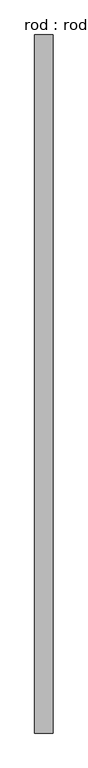
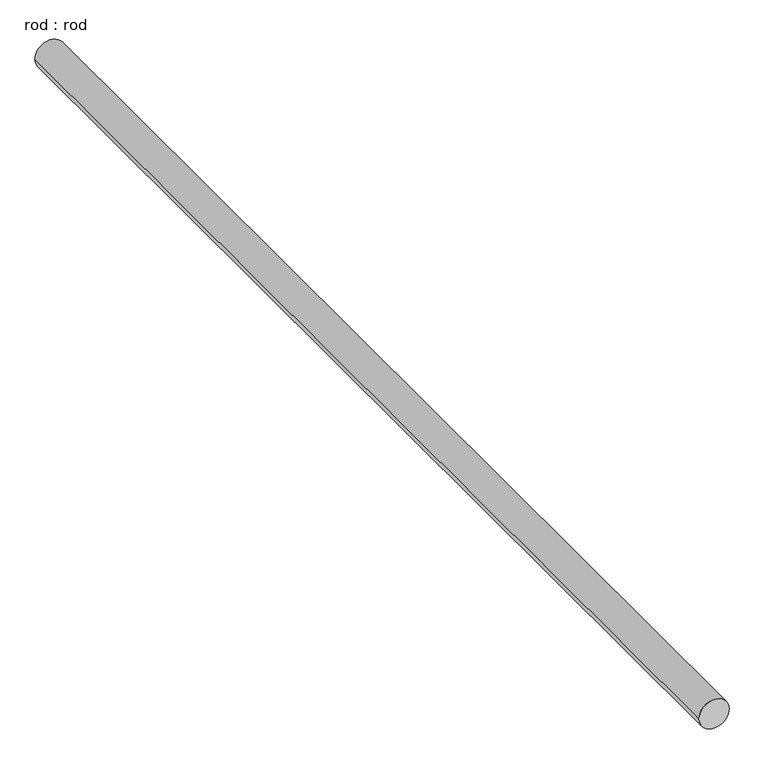
"""IFC4 building model written with IfcOpenShell, lengths in millimetres: proxy geometry, rod : rod."""

import ifcopenshell
import ifcopenshell.guid

model = None  # the IFC model being written
_history = None  # IfcOwnerHistory: only IFC2X3 demands one
_inside = {}  # id of a spatial element -> (the spatial element, [elements in it])
_under = {}  # id of a project, library or spatial element -> (it, [spatial elements below it])
_declared = {}  # id of a project -> (the project, [libraries it declares])
_typed = {}  # id of a type object -> (the type object, [elements of that type])
_made_of = {}  # id of a material, layer set ... -> (it, [elements and type objects made of it])


def new_model(schema):
    """Start an empty IFC model of exactly this schema.

    Asked for "IFC4X3", IfcOpenShell would pick the latest addendum, in which some entities
    have other attributes; the version numbers below select the first issue.
    IFC2X3 requires an IfcOwnerHistory on every rooted entity: one is made here for all.
    """
    global model, _history
    if schema == "IFC4X3":
        model = ifcopenshell.file(schema_version=(4, 3, 0, 0))
    else:
        model = ifcopenshell.file(schema=schema)
    _inside.clear()
    _under.clear()
    _declared.clear()
    _typed.clear()
    _made_of.clear()
    _history = None
    if model.schema == "IFC2X3":
        org = make("IfcOrganization", Name="unknown")
        user = make(
            "IfcPersonAndOrganization",
            ThePerson=make("IfcPerson", FamilyName="unknown"),
            TheOrganization=org,
        )
        app = make(
            "IfcApplication",
            ApplicationDeveloper=org,
            Version="unknown",
            ApplicationFullName="unknown",
            ApplicationIdentifier="unknown",
        )
        _history = make(
            "IfcOwnerHistory",
            OwningUser=user,
            OwningApplication=app,
            ChangeAction="ADDED",
            CreationDate=0,
        )
    return model


def make(cls, **values):
    """One entity of the class cls with the attributes given. An attribute that is None is left unset."""
    return model.create_entity(
        cls, **{name: value for name, value in values.items() if value is not None}
    )


def rooted(cls, **values):
    """An entity with a GlobalId (a new one), such as an element, a storey or a relation."""
    return make(cls, GlobalId=ifcopenshell.guid.new(), OwnerHistory=_history, **values)


def si_unit(unit_type, name, prefix=None):
    """IfcSIUnit, for example si_unit("LENGTHUNIT", "METRE", prefix="MILLI")."""
    return make("IfcSIUnit", UnitType=unit_type, Prefix=prefix, Name=name)


def assignment(units):
    """IfcUnitAssignment: the units of a project."""
    return None if units is None else make("IfcUnitAssignment", Units=units)


def point(xyz):
    """IfcCartesianPoint."""
    return None if xyz is None else make("IfcCartesianPoint", Coordinates=xyz)


def direction(xyz):
    """IfcDirection."""
    return None if xyz is None else make("IfcDirection", DirectionRatios=xyz)


def frame(location, z_axis=None, x_axis=None):
    """IfcAxis2Placement3D, a coordinate frame: its origin and axes. An axis left out is left unset."""
    return make(
        "IfcAxis2Placement3D",
        Location=point(location),
        Axis=direction(z_axis),
        RefDirection=direction(x_axis),
    )


def frame_2d(location, x_axis=None):
    """IfcAxis2Placement2D, a coordinate frame in the plane: its origin and x axis."""
    return make(
        "IfcAxis2Placement2D", Location=point(location), RefDirection=direction(x_axis)
    )


def origin():
    """The frame at (0, 0, 0) with its axes left unset."""
    return frame((0.0, 0.0, 0.0))


def place(relative_to, where):
    """IfcLocalPlacement: puts the frame where relative to a parent placement (None: the world)."""
    return make(
        "IfcLocalPlacement", PlacementRelTo=relative_to, RelativePlacement=where
    )


def context(
    kind, dimensions, precision=None, world=None, true_north=None, identifier=None
):
    """IfcGeometricRepresentationContext, for example the 3D "Model" context."""
    return make(
        "IfcGeometricRepresentationContext",
        ContextIdentifier=identifier,
        ContextType=kind,
        CoordinateSpaceDimension=dimensions,
        Precision=precision,
        WorldCoordinateSystem=world,
        TrueNorth=true_north,
    )


def project(units=None, contexts=None):
    """IfcProject with its units and contexts."""
    return rooted(
        "IfcProject",
        Name="project",
        RepresentationContexts=contexts,
        UnitsInContext=assignment(units),
    )


def spatial(cls, under=None, at=None, **own):
    """A site, building, storey or space (cls), placed at a placement, below another one or the project."""
    s = rooted(cls, ObjectPlacement=at, **own)
    if under is not None:
        _under.setdefault(under.id(), (under, []))[1].append(s)
    return s


def circle_curve(where, radius):
    """IfcCircle in the frame where."""
    return make("IfcCircle", Position=where, Radius=radius)


def trimmed(basis, trim1, trim2, sense, master):
    """IfcTrimmedCurve: the piece of a basis curve between two trims."""
    return make(
        "IfcTrimmedCurve",
        BasisCurve=basis,
        Trim1=trim1,
        Trim2=trim2,
        SenseAgreement=sense,
        MasterRepresentation=master,
    )


def segment(curve, same_sense, transition):
    """IfcCompositeCurveSegment."""
    return make(
        "IfcCompositeCurveSegment",
        Transition=transition,
        SameSense=same_sense,
        ParentCurve=curve,
    )


def composite_curve(segments, self_intersect=None):
    """IfcCompositeCurve: segments joined end to end."""
    return make("IfcCompositeCurve", Segments=segments, SelfIntersect=self_intersect)


def outline(outer, holes=None, kind="AREA"):
    """IfcArbitraryClosedProfileDef: a profile drawn as a closed curve; with holes, ...WithVoids."""
    if holes is None:
        return make("IfcArbitraryClosedProfileDef", ProfileType=kind, OuterCurve=outer)
    return make(
        "IfcArbitraryProfileDefWithVoids",
        ProfileType=kind,
        OuterCurve=outer,
        InnerCurves=holes,
    )


def extrude(swept, where, along, depth):
    """IfcExtrudedAreaSolid: the profile swept, set in the frame where, extruded along a direction by depth."""
    return make(
        "IfcExtrudedAreaSolid",
        SweptArea=swept,
        Position=where,
        ExtrudedDirection=direction(along),
        Depth=depth,
    )


def shape(context_of_items, identifier, shape_type, items):
    """IfcShapeRepresentation: the items that make up one representation, for example the "Body"."""
    return make(
        "IfcShapeRepresentation",
        ContextOfItems=context_of_items,
        RepresentationIdentifier=identifier,
        RepresentationType=shape_type,
        Items=items,
    )


def source(mapping_origin, context_of_items, identifier, shape_type, items):
    """IfcRepresentationMap: a shape defined once, which mapped items show again and again."""
    return make(
        "IfcRepresentationMap",
        MappingOrigin=mapping_origin,
        MappedRepresentation=shape(context_of_items, identifier, shape_type, items),
    )


def transform(
    local_origin,
    x_axis=None,
    y_axis=None,
    z_axis=None,
    scale=None,
    scale2=None,
    scale3=None,
    uniform=True,
):
    """IfcCartesianTransformationOperator3D, or its non-uniform kind. x_axis, y_axis, z_axis: its Axis1, 2, 3."""
    if uniform:
        return make(
            "IfcCartesianTransformationOperator3D",
            Axis1=direction(x_axis),
            Axis2=direction(y_axis),
            LocalOrigin=point(local_origin),
            Scale=scale,
            Axis3=direction(z_axis),
        )
    return make(
        "IfcCartesianTransformationOperator3DnonUniform",
        Axis1=direction(x_axis),
        Axis2=direction(y_axis),
        LocalOrigin=point(local_origin),
        Scale=scale,
        Axis3=direction(z_axis),
        Scale2=scale2,
        Scale3=scale3,
    )


def mapped(mapping_source, mapping_target):
    """IfcMappedItem: shows the shape of a source again, moved by a transform."""
    return make(
        "IfcMappedItem", MappingSource=mapping_source, MappingTarget=mapping_target
    )


def made_of(thing, what):
    """Note that an element or type object is made of a material, layer set ...; save() writes the relation."""
    if what is not None:
        _made_of.setdefault(what.id(), (what, []))[1].append(thing)
    return thing


def element(
    cls,
    number,
    at=None,
    inside=None,
    cuts=None,
    type_object=None,
    material=None,
    context=None,
    identifier="Body",
    shape_type=None,
    held_by="IfcProductDefinitionShape",
    body=None,
    shapes=None,
    **own,
):
    """One element of the class cls, such as IfcWall. Its Tag is "e" and its number.

    at: its placement. inside: the storey or other place that contains it. cuts: it is an
    opening in that element (IfcRelVoidsElement). A single representation is given by context,
    identifier, shape_type and body (its items); several are given by shapes. held_by: the class
    of the entity that holds the representations. save() writes the other relations.
    """
    e = rooted(cls, Tag="e%d" % number, ObjectPlacement=at, **own)
    if body is not None:
        shapes = [shape(context, identifier, shape_type, body)]
    if shapes is not None:
        e.Representation = make(held_by, Representations=shapes)
    if inside is not None:
        _inside.setdefault(inside.id(), (inside, []))[1].append(e)
    if cuts is not None:
        rooted(
            "IfcRelVoidsElement", RelatingBuildingElement=cuts, RelatedOpeningElement=e
        )
    if type_object is not None:
        _typed.setdefault(type_object.id(), (type_object, []))[1].append(e)
    return made_of(e, material)


def aggregate(whole, parts):
    """IfcRelAggregates: a whole, such as a stair, and the parts it consists of."""
    return rooted("IfcRelAggregates", RelatingObject=whole, RelatedObjects=parts)


def save(model, path):
    """Write the relations noted so far, then the file.

    IfcRelAggregates (storeys below a building ...), IfcRelContainedInSpatialStructure (elements
    in a storey), IfcRelDefinesByType, IfcRelAssociatesMaterial and IfcRelDeclares: one each for
    every whole, place, type object, material and project.
    """
    for whole, parts in _under.values():
        aggregate(whole, parts)
    for where, things in _inside.values():
        rooted(
            "IfcRelContainedInSpatialStructure",
            RelatedElements=things,
            RelatingStructure=where,
        )
    for kind, things in _typed.values():
        rooted("IfcRelDefinesByType", RelatedObjects=things, RelatingType=kind)
    for what, things in _made_of.values():
        rooted("IfcRelAssociatesMaterial", RelatedObjects=things, RelatingMaterial=what)
    for by, libraries in _declared.values():
        rooted("IfcRelDeclares", RelatingContext=by, RelatedDefinitions=libraries)
    model.write(path)


def rod_rod_8442bb91(model_context):
    return source(origin(), model_context, "Body", "SweptSolid", [
        extrude(outline(composite_curve([segment(trimmed(circle_curve(frame_2d((0.0108462, 0.0)), 200.0), [point((0.0108462, 200.0))], [point((0.0108462, -200.0))], False, "CARTESIAN"), True, "CONTINUOUS"), segment(trimmed(circle_curve(frame_2d((0.0108462, 0.0)), 200.0), [point((0.0108462, -200.0))], [point((0.0108462, 200.0))], False, "CARTESIAN"), True, "CONTINUOUS")], self_intersect=False)), frame((0.0, -3532.2713847, 0.0), z_axis=(0.0, 1.0, 0.0), x_axis=(0.0, 0.0, 1.0)), (0.0, 0.0, 1.0), 15250.0),
    ])


if __name__ == "__main__":
    model = new_model("IFC4")
    model_context = context("Model", 3, world=origin())
    ifc_project = project(units=[si_unit("LENGTHUNIT", "METRE", prefix="MILLI")], contexts=[model_context])
    site = spatial("IfcSite", under=ifc_project)
    building = spatial("IfcBuilding", under=site)
    placement = place(None, origin())
    rod_rod_shape = rod_rod_8442bb91(model_context)
    element("IfcBuildingElementProxy", 1, Name="rod : rod", ObjectType="rod : rod", at=placement, inside=building, context=model_context, shape_type="MappedRepresentation", body=[
        mapped(rod_rod_shape, transform((0.0, 0.0, 0.0), x_axis=(1.0, 0.0, 0.0), y_axis=(0.0, 1.0, 0.0), z_axis=(0.0, 0.0, 1.0))),
    ])
    save(model, "model.ifc")

# Revit data of these elements
# Type "rod : rod"
#   Default Elevation = 0
